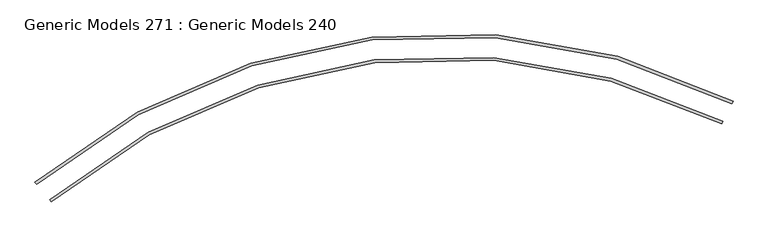
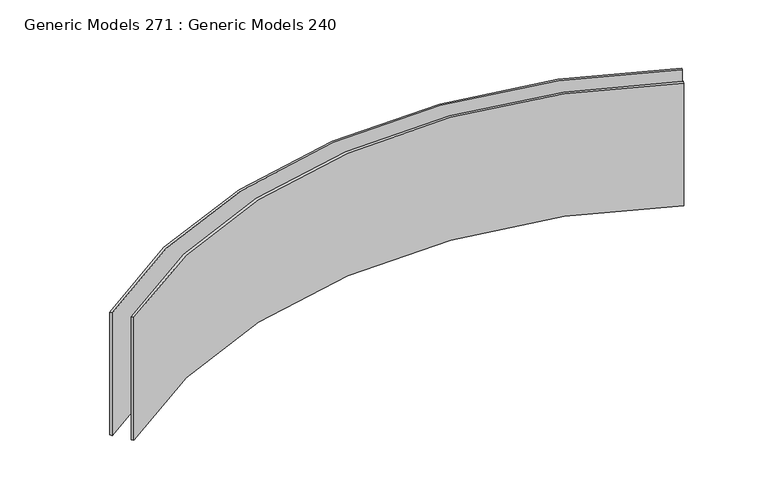
"""IFC4 building model written with IfcOpenShell, lengths in millimetres: proxy geometry, Generic Models 271 : Generic Models 240."""

from ifc_helpers import new_model, si_unit, point, frame, frame_2d, origin, place, context, project, spatial, polyline, circle_curve, trimmed, segment, composite_curve, outline, extrude, source, transform, mapped, element, save


def generic_models_271_generic_models_240_1e610eb9(model_context):
    return source(origin(), model_context, "Body", "SweptSolid", [
        extrude(outline(composite_curve([segment(trimmed(circle_curve(frame_2d((-832.04683, -25139.2753781)), 2947.0118053), [point((-2723.5515711, -22879.3885678))], [point((490.8431961, -22505.8668341))], False, "CARTESIAN"), True, "CONTINUOUS"), segment(polyline([(490.8431961, -22505.8668341), (485.1422677, -22517.2153765)]), True, "CONTINUOUS"), segment(trimmed(circle_curve(frame_2d((-832.04683, -25139.2753781)), 2934.3118053), [point((485.1422677, -22517.2153765))], [point((-2715.400226, -22889.127437))], True, "CARTESIAN"), True, "CONTINUOUS"), segment(polyline([(-2715.400226, -22889.127437), (-2723.5515711, -22879.3885678)]), True, "CONTINUOUS")], self_intersect=False)), frame((0.0, 0.0, 101.6), z_axis=(0.0, 0.0, 1.0), x_axis=(1.0, 0.0, 0.0)), (0.0, 0.0, 1.0), 679.45),
        extrude(outline(composite_curve([segment(trimmed(circle_curve(frame_2d((-832.04683, -25139.2753781)), 2842.1947981), [point((-2656.2760122, -22959.7664515))], [point((443.79168, -22599.5298461))], False, "CARTESIAN"), True, "CONTINUOUS"), segment(polyline([(443.79168, -22599.5298461), (438.0907516, -22610.8783886)]), True, "CONTINUOUS"), segment(trimmed(circle_curve(frame_2d((-832.04683, -25139.2753781)), 2829.4947981), [point((438.0907516, -22610.8783886))], [point((-2648.1246672, -22969.5053207))], True, "CARTESIAN"), True, "CONTINUOUS"), segment(polyline([(-2648.1246672, -22969.5053207), (-2656.2760122, -22959.7664515)]), True, "CONTINUOUS")], self_intersect=False)), frame((0.0, 0.0, 101.6), z_axis=(0.0, 0.0, 1.0), x_axis=(1.0, 0.0, 0.0)), (0.0, 0.0, 1.0), 679.45),
    ])


if __name__ == "__main__":
    model = new_model("IFC4")
    model_context = context("Model", 3, world=origin())
    ifc_project = project(units=[si_unit("LENGTHUNIT", "METRE", prefix="MILLI")], contexts=[model_context])
    site = spatial("IfcSite", under=ifc_project)
    building = spatial("IfcBuilding", under=site)
    placement = place(None, origin())
    generic_models_271_generic_models_240_shape = generic_models_271_generic_models_240_1e610eb9(model_context)
    element("IfcBuildingElementProxy", 1, Name="Generic Models 271 : Generic Models 240", ObjectType="Generic Models 271 : Generic Models 240", at=placement, inside=building, context=model_context, shape_type="MappedRepresentation", body=[
        mapped(generic_models_271_generic_models_240_shape, transform((0.0, 0.0, 0.0), x_axis=(1.0, 0.0, 0.0), y_axis=(0.0, 1.0, 0.0), z_axis=(0.0, 0.0, 1.0))),
    ])
    save(model, "model.ifc")

# Revit data of these elements
# Element 1 (IfcBuildingElementProxy, "Generic Models 271 : Generic Models 240")
#   Materials on its faces: "1/2\" GYP. BD", "PAINT - SHERWIN WILLLIAMS CORAL BELLS SW 6593"
# Materials
#   "1/2\" GYP. BD": class "Generic", colour RGB 171 170 168, transparency 0, Description = "Gypsum Wall Board", Cost = 0
#   "PAINT - SHERWIN WILLLIAMS CORAL BELLS SW 6593": class "Generic", colour RGB 148 56 61, transparency 0, Cost = 0
